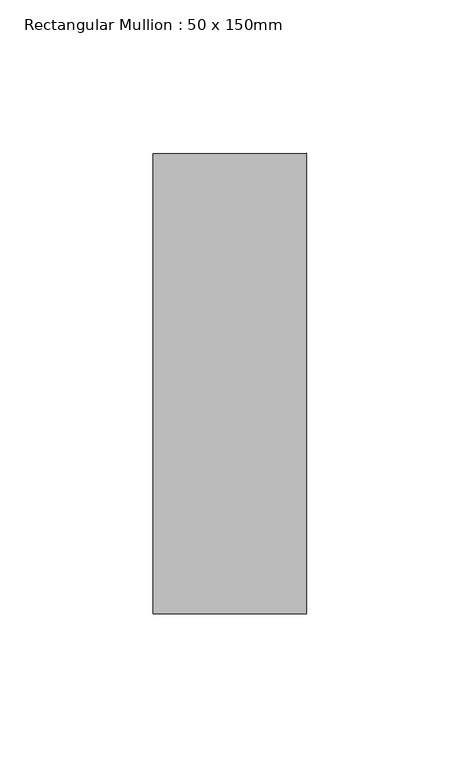
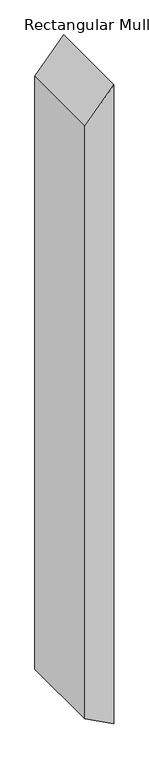
"""IFC4 building model written with IfcOpenShell, lengths in millimetres: member geometry, Rectangular Mullion : 50 x 150mm."""

import ifcopenshell
import ifcopenshell.guid

model = None  # the IFC model being written
_history = None  # IfcOwnerHistory: only IFC2X3 demands one
_inside = {}  # id of a spatial element -> (the spatial element, [elements in it])
_under = {}  # id of a project, library or spatial element -> (it, [spatial elements below it])
_declared = {}  # id of a project -> (the project, [libraries it declares])
_typed = {}  # id of a type object -> (the type object, [elements of that type])
_made_of = {}  # id of a material, layer set ... -> (it, [elements and type objects made of it])


def new_model(schema):
    """Start an empty IFC model of exactly this schema.

    Asked for "IFC4X3", IfcOpenShell would pick the latest addendum, in which some entities
    have other attributes; the version numbers below select the first issue.
    IFC2X3 requires an IfcOwnerHistory on every rooted entity: one is made here for all.
    """
    global model, _history
    if schema == "IFC4X3":
        model = ifcopenshell.file(schema_version=(4, 3, 0, 0))
    else:
        model = ifcopenshell.file(schema=schema)
    _inside.clear()
    _under.clear()
    _declared.clear()
    _typed.clear()
    _made_of.clear()
    _history = None
    if model.schema == "IFC2X3":
        org = make("IfcOrganization", Name="unknown")
        user = make(
            "IfcPersonAndOrganization",
            ThePerson=make("IfcPerson", FamilyName="unknown"),
            TheOrganization=org,
        )
        app = make(
            "IfcApplication",
            ApplicationDeveloper=org,
            Version="unknown",
            ApplicationFullName="unknown",
            ApplicationIdentifier="unknown",
        )
        _history = make(
            "IfcOwnerHistory",
            OwningUser=user,
            OwningApplication=app,
            ChangeAction="ADDED",
            CreationDate=0,
        )
    return model


def make(cls, **values):
    """One entity of the class cls with the attributes given. An attribute that is None is left unset."""
    return model.create_entity(
        cls, **{name: value for name, value in values.items() if value is not None}
    )


def rooted(cls, **values):
    """An entity with a GlobalId (a new one), such as an element, a storey or a relation."""
    return make(cls, GlobalId=ifcopenshell.guid.new(), OwnerHistory=_history, **values)


def si_unit(unit_type, name, prefix=None):
    """IfcSIUnit, for example si_unit("LENGTHUNIT", "METRE", prefix="MILLI")."""
    return make("IfcSIUnit", UnitType=unit_type, Prefix=prefix, Name=name)


def assignment(units):
    """IfcUnitAssignment: the units of a project."""
    return None if units is None else make("IfcUnitAssignment", Units=units)


def point(xyz):
    """IfcCartesianPoint."""
    return None if xyz is None else make("IfcCartesianPoint", Coordinates=xyz)


def direction(xyz):
    """IfcDirection."""
    return None if xyz is None else make("IfcDirection", DirectionRatios=xyz)


def frame(location, z_axis=None, x_axis=None):
    """IfcAxis2Placement3D, a coordinate frame: its origin and axes. An axis left out is left unset."""
    return make(
        "IfcAxis2Placement3D",
        Location=point(location),
        Axis=direction(z_axis),
        RefDirection=direction(x_axis),
    )


def origin():
    """The frame at (0, 0, 0) with its axes left unset."""
    return frame((0.0, 0.0, 0.0))


def place(relative_to, where):
    """IfcLocalPlacement: puts the frame where relative to a parent placement (None: the world)."""
    return make(
        "IfcLocalPlacement", PlacementRelTo=relative_to, RelativePlacement=where
    )


def context(
    kind, dimensions, precision=None, world=None, true_north=None, identifier=None
):
    """IfcGeometricRepresentationContext, for example the 3D "Model" context."""
    return make(
        "IfcGeometricRepresentationContext",
        ContextIdentifier=identifier,
        ContextType=kind,
        CoordinateSpaceDimension=dimensions,
        Precision=precision,
        WorldCoordinateSystem=world,
        TrueNorth=true_north,
    )


def project(units=None, contexts=None):
    """IfcProject with its units and contexts."""
    return rooted(
        "IfcProject",
        Name="project",
        RepresentationContexts=contexts,
        UnitsInContext=assignment(units),
    )


def spatial(cls, under=None, at=None, **own):
    """A site, building, storey or space (cls), placed at a placement, below another one or the project."""
    s = rooted(cls, ObjectPlacement=at, **own)
    if under is not None:
        _under.setdefault(under.id(), (under, []))[1].append(s)
    return s


def polyline(points):
    """IfcPolyline through the points."""
    return make("IfcPolyline", Points=[point(p) for p in points])


def outline(outer, holes=None, kind="AREA"):
    """IfcArbitraryClosedProfileDef: a profile drawn as a closed curve; with holes, ...WithVoids."""
    if holes is None:
        return make("IfcArbitraryClosedProfileDef", ProfileType=kind, OuterCurve=outer)
    return make(
        "IfcArbitraryProfileDefWithVoids",
        ProfileType=kind,
        OuterCurve=outer,
        InnerCurves=holes,
    )


def extrude(swept, where, along, depth):
    """IfcExtrudedAreaSolid: the profile swept, set in the frame where, extruded along a direction by depth."""
    return make(
        "IfcExtrudedAreaSolid",
        SweptArea=swept,
        Position=where,
        ExtrudedDirection=direction(along),
        Depth=depth,
    )


def shape(context_of_items, identifier, shape_type, items):
    """IfcShapeRepresentation: the items that make up one representation, for example the "Body"."""
    return make(
        "IfcShapeRepresentation",
        ContextOfItems=context_of_items,
        RepresentationIdentifier=identifier,
        RepresentationType=shape_type,
        Items=items,
    )


def source(mapping_origin, context_of_items, identifier, shape_type, items):
    """IfcRepresentationMap: a shape defined once, which mapped items show again and again."""
    return make(
        "IfcRepresentationMap",
        MappingOrigin=mapping_origin,
        MappedRepresentation=shape(context_of_items, identifier, shape_type, items),
    )


def transform(
    local_origin,
    x_axis=None,
    y_axis=None,
    z_axis=None,
    scale=None,
    scale2=None,
    scale3=None,
    uniform=True,
):
    """IfcCartesianTransformationOperator3D, or its non-uniform kind. x_axis, y_axis, z_axis: its Axis1, 2, 3."""
    if uniform:
        return make(
            "IfcCartesianTransformationOperator3D",
            Axis1=direction(x_axis),
            Axis2=direction(y_axis),
            LocalOrigin=point(local_origin),
            Scale=scale,
            Axis3=direction(z_axis),
        )
    return make(
        "IfcCartesianTransformationOperator3DnonUniform",
        Axis1=direction(x_axis),
        Axis2=direction(y_axis),
        LocalOrigin=point(local_origin),
        Scale=scale,
        Axis3=direction(z_axis),
        Scale2=scale2,
        Scale3=scale3,
    )


def mapped(mapping_source, mapping_target):
    """IfcMappedItem: shows the shape of a source again, moved by a transform."""
    return make(
        "IfcMappedItem", MappingSource=mapping_source, MappingTarget=mapping_target
    )


def made_of(thing, what):
    """Note that an element or type object is made of a material, layer set ...; save() writes the relation."""
    if what is not None:
        _made_of.setdefault(what.id(), (what, []))[1].append(thing)
    return thing


def element(
    cls,
    number,
    at=None,
    inside=None,
    cuts=None,
    type_object=None,
    material=None,
    context=None,
    identifier="Body",
    shape_type=None,
    held_by="IfcProductDefinitionShape",
    body=None,
    shapes=None,
    **own,
):
    """One element of the class cls, such as IfcWall. Its Tag is "e" and its number.

    at: its placement. inside: the storey or other place that contains it. cuts: it is an
    opening in that element (IfcRelVoidsElement). A single representation is given by context,
    identifier, shape_type and body (its items); several are given by shapes. held_by: the class
    of the entity that holds the representations. save() writes the other relations.
    """
    e = rooted(cls, Tag="e%d" % number, ObjectPlacement=at, **own)
    if body is not None:
        shapes = [shape(context, identifier, shape_type, body)]
    if shapes is not None:
        e.Representation = make(held_by, Representations=shapes)
    if inside is not None:
        _inside.setdefault(inside.id(), (inside, []))[1].append(e)
    if cuts is not None:
        rooted(
            "IfcRelVoidsElement", RelatingBuildingElement=cuts, RelatedOpeningElement=e
        )
    if type_object is not None:
        _typed.setdefault(type_object.id(), (type_object, []))[1].append(e)
    return made_of(e, material)


def aggregate(whole, parts):
    """IfcRelAggregates: a whole, such as a stair, and the parts it consists of."""
    return rooted("IfcRelAggregates", RelatingObject=whole, RelatedObjects=parts)


def save(model, path):
    """Write the relations noted so far, then the file.

    IfcRelAggregates (storeys below a building ...), IfcRelContainedInSpatialStructure (elements
    in a storey), IfcRelDefinesByType, IfcRelAssociatesMaterial and IfcRelDeclares: one each for
    every whole, place, type object, material and project.
    """
    for whole, parts in _under.values():
        aggregate(whole, parts)
    for where, things in _inside.values():
        rooted(
            "IfcRelContainedInSpatialStructure",
            RelatedElements=things,
            RelatingStructure=where,
        )
    for kind, things in _typed.values():
        rooted("IfcRelDefinesByType", RelatedObjects=things, RelatingType=kind)
    for what, things in _made_of.values():
        rooted("IfcRelAssociatesMaterial", RelatedObjects=things, RelatingMaterial=what)
    for by, libraries in _declared.values():
        rooted("IfcRelDeclares", RelatingContext=by, RelatedDefinitions=libraries)
    model.write(path)


def rectangular_mullion_50_x_150mm_a1f019ed(model_context):
    return source(origin(), model_context, "Body", "SweptSolid", [
        extrude(outline(polyline([(0.0, 0.0), (-58.5251446, -50.0), (-1143.6098029, -50.0), (-1169.4475431, 0.0), (0.0, 0.0)])), frame((0.0, -75.0, 0.0), z_axis=(0.0, 1.0, 0.0), x_axis=(0.0, 0.0, 1.0)), (0.0, 0.0, 1.0), 150.0),
    ])


if __name__ == "__main__":
    model = new_model("IFC4")
    model_context = context("Model", 3, world=origin())
    ifc_project = project(units=[si_unit("LENGTHUNIT", "METRE", prefix="MILLI")], contexts=[model_context])
    site = spatial("IfcSite", under=ifc_project)
    building = spatial("IfcBuilding", under=site)
    placement = place(None, origin())
    rectangular_mullion_50_x_150mm_shape = rectangular_mullion_50_x_150mm_a1f019ed(model_context)
    element("IfcMember", 1, ObjectType="Rectangular Mullion : 50 x 150mm", at=placement, inside=building, context=model_context, shape_type="MappedRepresentation", body=[
        mapped(rectangular_mullion_50_x_150mm_shape, transform((0.0, 0.0, 0.0), x_axis=(1.0, 0.0, 0.0), y_axis=(0.0, 1.0, 0.0), z_axis=(0.0, 0.0, 1.0))),
    ])
    save(model, "model.ifc")

# Revit data of these elements
# Type "Rectangular Mullion : 50 x 150mm"
#   built-in parameter 1007304 = 0.492126 (stored number, unit not read)
#   built-in parameter 1007301 = 0.082021 (stored number, unit not read)
#   built-in parameter 1007300 = 0.082021 (stored number, unit not read)
# Element 1 (IfcMember, "Rectangular Mullion : 50 x 150mm")
#   Materials on its faces: "Metal - Aluminium"
# Materials
#   "Metal - Aluminium": class "Metal", colour RGB 247 247 247, transparency 0
